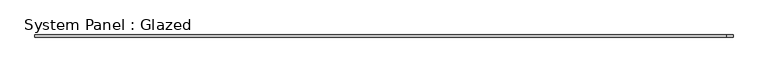
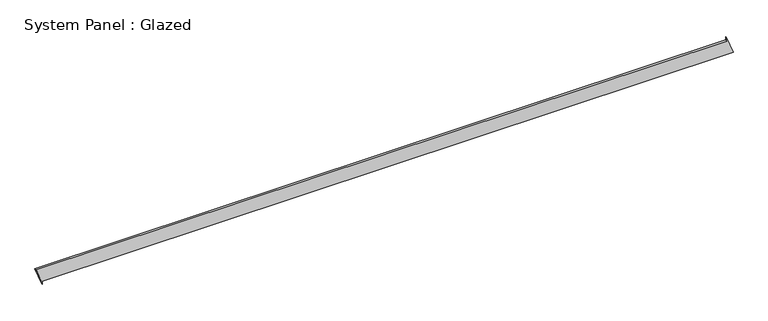
"""IFC4 building model written with IfcOpenShell, lengths in millimetres: plate geometry, System Panel : Glazed."""

import ifcopenshell
import ifcopenshell.guid

model = None  # the IFC model being written
_history = None  # IfcOwnerHistory: only IFC2X3 demands one
_inside = {}  # id of a spatial element -> (the spatial element, [elements in it])
_under = {}  # id of a project, library or spatial element -> (it, [spatial elements below it])
_declared = {}  # id of a project -> (the project, [libraries it declares])
_typed = {}  # id of a type object -> (the type object, [elements of that type])
_made_of = {}  # id of a material, layer set ... -> (it, [elements and type objects made of it])


def new_model(schema):
    """Start an empty IFC model of exactly this schema.

    Asked for "IFC4X3", IfcOpenShell would pick the latest addendum, in which some entities
    have other attributes; the version numbers below select the first issue.
    IFC2X3 requires an IfcOwnerHistory on every rooted entity: one is made here for all.
    """
    global model, _history
    if schema == "IFC4X3":
        model = ifcopenshell.file(schema_version=(4, 3, 0, 0))
    else:
        model = ifcopenshell.file(schema=schema)
    _inside.clear()
    _under.clear()
    _declared.clear()
    _typed.clear()
    _made_of.clear()
    _history = None
    if model.schema == "IFC2X3":
        org = make("IfcOrganization", Name="unknown")
        user = make(
            "IfcPersonAndOrganization",
            ThePerson=make("IfcPerson", FamilyName="unknown"),
            TheOrganization=org,
        )
        app = make(
            "IfcApplication",
            ApplicationDeveloper=org,
            Version="unknown",
            ApplicationFullName="unknown",
            ApplicationIdentifier="unknown",
        )
        _history = make(
            "IfcOwnerHistory",
            OwningUser=user,
            OwningApplication=app,
            ChangeAction="ADDED",
            CreationDate=0,
        )
    return model


def make(cls, **values):
    """One entity of the class cls with the attributes given. An attribute that is None is left unset."""
    return model.create_entity(
        cls, **{name: value for name, value in values.items() if value is not None}
    )


def rooted(cls, **values):
    """An entity with a GlobalId (a new one), such as an element, a storey or a relation."""
    return make(cls, GlobalId=ifcopenshell.guid.new(), OwnerHistory=_history, **values)


def si_unit(unit_type, name, prefix=None):
    """IfcSIUnit, for example si_unit("LENGTHUNIT", "METRE", prefix="MILLI")."""
    return make("IfcSIUnit", UnitType=unit_type, Prefix=prefix, Name=name)


def assignment(units):
    """IfcUnitAssignment: the units of a project."""
    return None if units is None else make("IfcUnitAssignment", Units=units)


def point(xyz):
    """IfcCartesianPoint."""
    return None if xyz is None else make("IfcCartesianPoint", Coordinates=xyz)


def direction(xyz):
    """IfcDirection."""
    return None if xyz is None else make("IfcDirection", DirectionRatios=xyz)


def frame(location, z_axis=None, x_axis=None):
    """IfcAxis2Placement3D, a coordinate frame: its origin and axes. An axis left out is left unset."""
    return make(
        "IfcAxis2Placement3D",
        Location=point(location),
        Axis=direction(z_axis),
        RefDirection=direction(x_axis),
    )


def origin():
    """The frame at (0, 0, 0) with its axes left unset."""
    return frame((0.0, 0.0, 0.0))


def place(relative_to, where):
    """IfcLocalPlacement: puts the frame where relative to a parent placement (None: the world)."""
    return make(
        "IfcLocalPlacement", PlacementRelTo=relative_to, RelativePlacement=where
    )


def context(
    kind, dimensions, precision=None, world=None, true_north=None, identifier=None
):
    """IfcGeometricRepresentationContext, for example the 3D "Model" context."""
    return make(
        "IfcGeometricRepresentationContext",
        ContextIdentifier=identifier,
        ContextType=kind,
        CoordinateSpaceDimension=dimensions,
        Precision=precision,
        WorldCoordinateSystem=world,
        TrueNorth=true_north,
    )


def project(units=None, contexts=None):
    """IfcProject with its units and contexts."""
    return rooted(
        "IfcProject",
        Name="project",
        RepresentationContexts=contexts,
        UnitsInContext=assignment(units),
    )


def spatial(cls, under=None, at=None, **own):
    """A site, building, storey or space (cls), placed at a placement, below another one or the project."""
    s = rooted(cls, ObjectPlacement=at, **own)
    if under is not None:
        _under.setdefault(under.id(), (under, []))[1].append(s)
    return s


def polyline(points):
    """IfcPolyline through the points."""
    return make("IfcPolyline", Points=[point(p) for p in points])


def outline(outer, holes=None, kind="AREA"):
    """IfcArbitraryClosedProfileDef: a profile drawn as a closed curve; with holes, ...WithVoids."""
    if holes is None:
        return make("IfcArbitraryClosedProfileDef", ProfileType=kind, OuterCurve=outer)
    return make(
        "IfcArbitraryProfileDefWithVoids",
        ProfileType=kind,
        OuterCurve=outer,
        InnerCurves=holes,
    )


def extrude(swept, where, along, depth):
    """IfcExtrudedAreaSolid: the profile swept, set in the frame where, extruded along a direction by depth."""
    return make(
        "IfcExtrudedAreaSolid",
        SweptArea=swept,
        Position=where,
        ExtrudedDirection=direction(along),
        Depth=depth,
    )


def shape(context_of_items, identifier, shape_type, items):
    """IfcShapeRepresentation: the items that make up one representation, for example the "Body"."""
    return make(
        "IfcShapeRepresentation",
        ContextOfItems=context_of_items,
        RepresentationIdentifier=identifier,
        RepresentationType=shape_type,
        Items=items,
    )


def source(mapping_origin, context_of_items, identifier, shape_type, items):
    """IfcRepresentationMap: a shape defined once, which mapped items show again and again."""
    return make(
        "IfcRepresentationMap",
        MappingOrigin=mapping_origin,
        MappedRepresentation=shape(context_of_items, identifier, shape_type, items),
    )


def transform(
    local_origin,
    x_axis=None,
    y_axis=None,
    z_axis=None,
    scale=None,
    scale2=None,
    scale3=None,
    uniform=True,
):
    """IfcCartesianTransformationOperator3D, or its non-uniform kind. x_axis, y_axis, z_axis: its Axis1, 2, 3."""
    if uniform:
        return make(
            "IfcCartesianTransformationOperator3D",
            Axis1=direction(x_axis),
            Axis2=direction(y_axis),
            LocalOrigin=point(local_origin),
            Scale=scale,
            Axis3=direction(z_axis),
        )
    return make(
        "IfcCartesianTransformationOperator3DnonUniform",
        Axis1=direction(x_axis),
        Axis2=direction(y_axis),
        LocalOrigin=point(local_origin),
        Scale=scale,
        Axis3=direction(z_axis),
        Scale2=scale2,
        Scale3=scale3,
    )


def mapped(mapping_source, mapping_target):
    """IfcMappedItem: shows the shape of a source again, moved by a transform."""
    return make(
        "IfcMappedItem", MappingSource=mapping_source, MappingTarget=mapping_target
    )


def made_of(thing, what):
    """Note that an element or type object is made of a material, layer set ...; save() writes the relation."""
    if what is not None:
        _made_of.setdefault(what.id(), (what, []))[1].append(thing)
    return thing


def element(
    cls,
    number,
    at=None,
    inside=None,
    cuts=None,
    type_object=None,
    material=None,
    context=None,
    identifier="Body",
    shape_type=None,
    held_by="IfcProductDefinitionShape",
    body=None,
    shapes=None,
    **own,
):
    """One element of the class cls, such as IfcWall. Its Tag is "e" and its number.

    at: its placement. inside: the storey or other place that contains it. cuts: it is an
    opening in that element (IfcRelVoidsElement). A single representation is given by context,
    identifier, shape_type and body (its items); several are given by shapes. held_by: the class
    of the entity that holds the representations. save() writes the other relations.
    """
    e = rooted(cls, Tag="e%d" % number, ObjectPlacement=at, **own)
    if body is not None:
        shapes = [shape(context, identifier, shape_type, body)]
    if shapes is not None:
        e.Representation = make(held_by, Representations=shapes)
    if inside is not None:
        _inside.setdefault(inside.id(), (inside, []))[1].append(e)
    if cuts is not None:
        rooted(
            "IfcRelVoidsElement", RelatingBuildingElement=cuts, RelatedOpeningElement=e
        )
    if type_object is not None:
        _typed.setdefault(type_object.id(), (type_object, []))[1].append(e)
    return made_of(e, material)


def aggregate(whole, parts):
    """IfcRelAggregates: a whole, such as a stair, and the parts it consists of."""
    return rooted("IfcRelAggregates", RelatingObject=whole, RelatedObjects=parts)


def save(model, path):
    """Write the relations noted so far, then the file.

    IfcRelAggregates (storeys below a building ...), IfcRelContainedInSpatialStructure (elements
    in a storey), IfcRelDefinesByType, IfcRelAssociatesMaterial and IfcRelDeclares: one each for
    every whole, place, type object, material and project.
    """
    for whole, parts in _under.values():
        aggregate(whole, parts)
    for where, things in _inside.values():
        rooted(
            "IfcRelContainedInSpatialStructure",
            RelatedElements=things,
            RelatingStructure=where,
        )
    for kind, things in _typed.values():
        rooted("IfcRelDefinesByType", RelatedObjects=things, RelatingType=kind)
    for what, things in _made_of.values():
        rooted("IfcRelAssociatesMaterial", RelatedObjects=things, RelatingMaterial=what)
    for by, libraries in _declared.values():
        rooted("IfcRelDeclares", RelatingContext=by, RelatedDefinitions=libraries)
    model.write(path)


def system_panel_glazed_7ff1da7a(model_context):
    return source(origin(), model_context, "Body", "SweptSolid", [
        extrude(outline(polyline([(0.0, -3956.991033), (35.3553391, -3956.991033), (35.3553391, 4027.528574), (233.766037, 3956.5208191), (198.410698, 3956.5199259), (198.6124026, -4027.528574), (0.0, -3956.991033)])), frame((0.0, -49.5, 0.0), z_axis=(0.0, 1.0, 0.0), x_axis=(0.0, 0.0, 1.0)), (0.0, 0.0, 1.0), 25.0),
    ])


if __name__ == "__main__":
    model = new_model("IFC4")
    model_context = context("Model", 3, world=origin())
    ifc_project = project(units=[si_unit("LENGTHUNIT", "METRE", prefix="MILLI")], contexts=[model_context])
    site = spatial("IfcSite", under=ifc_project)
    building = spatial("IfcBuilding", under=site)
    placement = place(None, origin())
    system_panel_glazed_shape = system_panel_glazed_7ff1da7a(model_context)
    element("IfcPlate", 1, ObjectType="System Panel : Glazed", at=placement, inside=building, context=model_context, shape_type="MappedRepresentation", body=[
        mapped(system_panel_glazed_shape, transform((0.0, 0.0, 0.0), x_axis=(1.0, 0.0, 0.0), y_axis=(0.0, 1.0, 0.0), z_axis=(0.0, 0.0, 1.0))),
    ])
    save(model, "model.ifc")

# Revit data of these elements
# Element 1 (IfcPlate, "System Panel : Glazed")
#   Materials on its faces: "Glass"
# Materials
#   "Glass": class "Glass", colour RGB 218 227 224, transparency 0.85, Description = "Soda Lime Glass", Cost = 0
